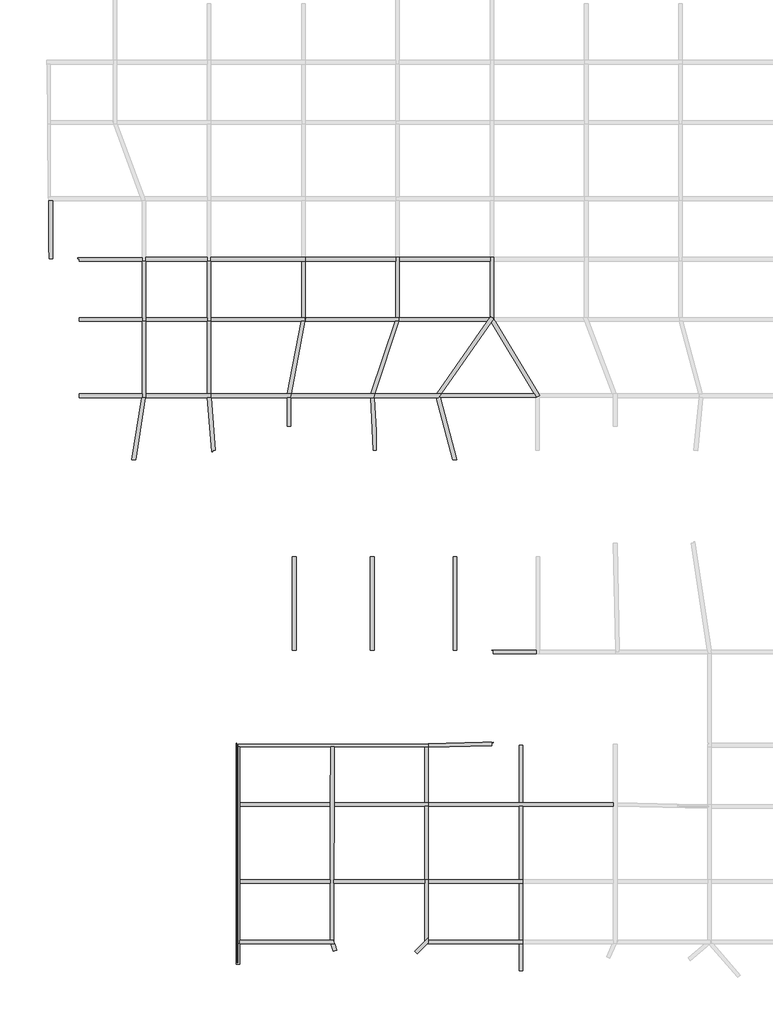
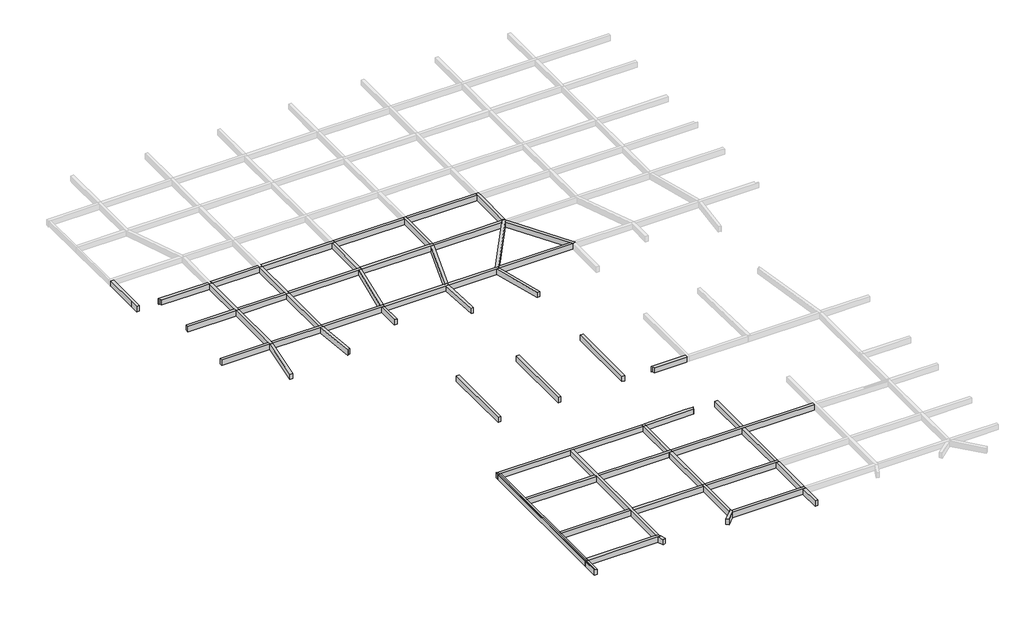
# One storey, part 1 of 15: 57 beams.
"""IFC4 building model written with IfcOpenShell, lengths in millimetres."""

from ifc_helpers import new_model, si_unit, frame, origin, place, context, project, spatial, polyline, outline, extrude, faceted_brep, element, save

model = new_model("IFC4")

# Units and contexts
model_context = context("Model", 3, world=origin())
ifc_project = project(units=[si_unit("LENGTHUNIT", "METRE", prefix="MILLI")], contexts=[model_context])

# Site, building, storey
site = spatial("IfcSite", under=ifc_project)
building = spatial("IfcBuilding", under=site)
storey = spatial("IfcBuildingStorey", under=building, Name="层高", Elevation=3300.0)

# Beams
placement = place(None, origin())
element("IfcBeam", 1, ObjectType="混凝土 - 矩形梁 : KL_beam", at=placement, inside=storey, context=model_context, shape_type="Brep", body=[
    faceted_brep([(117908.7029725, 38177.5268795, 3300.0), (117908.7029725, 38177.5268795, 2700.0), (118120.8350069, 37965.3948451, 2700.0), (118120.8350069, 37965.3948451, 3300.0), (118962.3353106, 38806.8951488, 3300.0), (119050.2032763, 38894.7631145, 3300.0), (119050.2032763, 39106.8951488, 3300.0), (119050.2032763, 39319.0271832, 3300.0), (118750.2032763, 39019.0271832, 3300.0), (118962.3353106, 38806.8951488, 2700.0), (119050.2032763, 38894.7631145, 2700.0), (118750.2032763, 39019.0271832, 2700.0), (119050.2032763, 39319.0271832, 2700.0), (119050.2032763, 39106.8951488, 2700.0)], [[[0, 1, 2, 3]], [[0, 3, 4, 5, 6, 7, 8]], [[3, 2, 9, 10, 5, 4]], [[2, 1, 11, 12, 13, 10, 9]], [[1, 0, 8, 7, 12, 11]], [[7, 6, 5, 10, 13, 12]]]),
])
element("IfcBeam", 2, ObjectType="混凝土 - 矩形梁 : KL_beam", at=placement, inside=storey, context=model_context, shape_type="Brep", body=[
    faceted_brep([(119050.2032763, 44092.5925365, 3300.0), (118750.2032763, 44092.5925365, 3300.0), (118750.2032763, 43792.5925365, 3300.0), (118750.2032763, 39019.0271832, 3300.0), (119050.2032763, 39319.0271832, 3300.0), (119050.2032763, 43792.5925365, 3300.0), (119050.2032763, 44092.5925365, 2700.0), (119050.2032763, 39319.0271832, 2700.0), (119050.2032763, 43792.5925365, 2700.0), (118750.2032763, 44092.5925365, 2700.0), (118750.2032763, 39019.0271832, 2700.0), (118750.2032763, 43792.5925365, 2700.0)], [[[0, 1, 2, 3, 4, 5]], [[6, 0, 5, 4, 7, 8]], [[9, 6, 8, 7, 10, 11]], [[1, 9, 11, 10, 3, 2]], [[4, 3, 10, 7]], [[1, 0, 6, 9]]]),
])
element("IfcBeam", 3, ObjectType="混凝土 - 矩形梁 : KL_beam", at=placement, inside=storey, context=model_context, shape_type="Brep", body=[
    faceted_brep([(118962.3353106, 38806.8951488, 3300.0), (118962.3353106, 38806.8951488, 2700.0), (126550.2032763, 38806.8951488, 2700.0), (126850.2032763, 38806.8951488, 2700.0), (126850.2032763, 38806.8951488, 3300.0), (126550.2032763, 38806.8951488, 3300.0), (119050.2032763, 38894.7631145, 3300.0), (119050.2032763, 38894.7631145, 2700.0), (119050.2032763, 39106.8951488, 3300.0), (119050.2032763, 39106.8951488, 2700.0), (126850.2032763, 39106.8951488, 3300.0), (126550.2032763, 39106.8951488, 3300.0), (126550.2032763, 39106.8951488, 2700.0), (126850.2032763, 39106.8951488, 2700.0)], [[[0, 1, 2, 3, 4, 5]], [[6, 7, 1, 0]], [[7, 6, 8, 9]], [[6, 0, 5, 4, 10, 11, 8]], [[1, 7, 9, 12, 13, 3, 2]], [[9, 8, 11, 10, 13, 12]], [[10, 4, 3, 13]]]),
])
element("IfcBeam", 4, ObjectType="混凝土 - 矩形梁 : KL_beam", at=placement, inside=storey, context=model_context, shape_type="Brep", body=[
    faceted_brep([(103150.2032763, 55392.5925366, 3300.0), (103150.2032763, 55092.5925366, 3300.0), (103172.8784474, 55092.5925366, 3300.0), (103172.8784474, 55392.5925366, 3300.0), (103150.2032763, 55392.5925366, 2700.0), (103172.8784474, 55392.5925366, 2700.0), (103150.2032763, 55092.5925366, 2700.0), (103172.8784474, 55092.5925366, 2700.0)], [[[0, 1, 2, 3]], [[4, 0, 3, 5]], [[6, 4, 5, 7]], [[1, 6, 7, 2]], [[1, 0, 4, 6]], [[3, 2, 7, 5]]]),
    faceted_brep([(119050.2032763, 55092.5925366, 3300.0), (119050.2032763, 55092.5925366, 2700.0), (119050.2032763, 55336.6611358, 2700.0), (119050.2032763, 55336.6611358, 3300.0), (103292.8784474, 55092.5925366, 2700.0), (103292.8784474, 55092.5925366, 3300.0), (103292.8784474, 55332.5925366, 3300.0), (103292.8784474, 55332.5925366, 2700.0), (103450.2032763, 55092.5925366, 3300.0), (110949.9406263, 55092.5925366, 3300.0), (111249.9410854, 55092.5925366, 3300.0), (118901.021306, 55332.5925366, 3300.0), (118901.021306, 55332.5925366, 2700.0), (111249.9410854, 55092.5925366, 2700.0), (110949.9406263, 55092.5925366, 2700.0), (103450.2032763, 55092.5925366, 2700.0)], [[[0, 1, 2, 3]], [[4, 5, 6, 7]], [[6, 5, 8, 9, 10, 0, 3, 11]], [[4, 7, 12, 2, 1, 13, 14, 15]], [[1, 0, 10, 9, 8, 5, 4, 15, 14, 13]], [[7, 6, 11, 12]], [[3, 2, 12, 11]]]),
])
element("IfcBeam", 5, ObjectType="混凝土 - 矩形梁 : KL_beam", at=placement, inside=storey, context=model_context, shape_type="Brep", body=[
    faceted_brep([(103450.2032763, 38806.8951488, 3300.0), (103450.2032763, 39106.8951488, 3300.0), (103450.2032763, 43792.5925365, 3300.0), (103450.2032763, 44092.5925365, 3300.0), (103450.2032763, 50192.5925366, 3300.0), (103450.2032763, 50492.5925366, 3300.0), (103450.2032763, 55092.5925366, 3300.0), (103292.8784474, 55092.5925366, 3300.0), (103292.8784474, 38806.8951488, 3300.0), (103450.2032763, 55092.5925366, 2700.0), (103450.2032763, 38806.8951488, 2700.0), (103450.2032763, 39106.8951488, 2700.0), (103450.2032763, 43792.5925365, 2700.0), (103450.2032763, 44092.5925365, 2700.0), (103450.2032763, 50192.5925366, 2700.0), (103450.2032763, 50492.5925366, 2700.0), (103292.8784474, 55092.5925366, 2700.0), (103292.8784474, 38806.8951488, 2700.0)], [[[0, 1, 2, 3, 4, 5, 6, 7, 8]], [[9, 6, 5, 4, 3, 2, 1, 0, 10, 11, 12, 13, 14, 15]], [[8, 7, 16, 17]], [[9, 15, 14, 13, 12, 11, 10, 17, 16]], [[6, 9, 16, 7]], [[10, 0, 8, 17]]]),
    faceted_brep([(103150.2032763, 55092.5925366, 3300.0), (103150.2032763, 55092.5925366, 2700.0), (103150.2032763, 38806.8951488, 2700.0), (103150.2032763, 38806.8951488, 3300.0), (103172.8784474, 55092.5925366, 2700.0), (103172.8784474, 38806.8951488, 2700.0), (103172.8784474, 55092.5925366, 3300.0), (103172.8784474, 38806.8951488, 3300.0)], [[[0, 1, 2, 3]], [[2, 1, 4, 5]], [[1, 0, 6, 4]], [[3, 2, 5, 7]], [[6, 7, 5, 4]], [[0, 3, 7, 6]]]),
])
element("IfcBeam", 6, ObjectType="混凝土 - 矩形梁 : KL_beam", at=placement, inside=storey, context=model_context, shape_type="SweptSolid", body=[
    extrude(outline(polyline([(103450.2032763, 37131.5943874), (103150.2032763, 37131.5943874), (103150.2032763, 38806.8951488), (103172.8784474, 38806.8951488), (103172.8784474, 37194.4264136), (103292.8784474, 37191.4907698), (103292.8784474, 38806.8951488), (103450.2032763, 38806.8951488), (103450.2032763, 37131.5943874)])), frame((0.0, 0.0, 2700.0), z_axis=(0.0, 0.0, 1.0), x_axis=(1.0, 0.0, 0.0)), (0.0, 0.0, 1.0), 600.0),
])
element("IfcBeam", 7, ObjectType="混凝土 - 矩形梁 : KL_beam", at=placement, inside=storey, context=model_context, shape_type="Brep", body=[
    faceted_brep([(111284.8038396, 38806.8951488, 3300.0), (111221.7575553, 38982.8323121, 3300.0), (111177.3002006, 39106.8951488, 3300.0), (110921.9741403, 39106.8951488, 3300.0), (103450.2032763, 39106.8951488, 3300.0), (103450.2032763, 38806.8951488, 3300.0), (110966.1236984, 38806.8951488, 3300.0), (111284.8038396, 38806.8951488, 2700.0), (103450.2032763, 38806.8951488, 2700.0), (110966.1236984, 38806.8951488, 2700.0), (111177.3002006, 39106.8951488, 2700.0), (111221.7575553, 38982.8323121, 2700.0), (103450.2032763, 39106.8951488, 2700.0), (110921.9741403, 39106.8951488, 2700.0)], [[[0, 1, 2, 3, 4, 5, 6]], [[7, 0, 6, 5, 8, 9]], [[10, 11, 7, 9, 8, 12, 13]], [[2, 10, 13, 12, 4, 3]], [[5, 4, 12, 8]], [[2, 1, 0, 7, 11, 10]]]),
])
element("IfcBeam", 8, ObjectType="混凝土 - 矩形梁 : KL_beam", at=placement, inside=storey, context=model_context, shape_type="SweptSolid", body=[
    extrude(outline(polyline([(111471.66124, 38285.4502876), (111189.2464034, 38184.2482122), (110966.1236984, 38806.8951488), (111284.8038396, 38806.8951488), (111471.66124, 38285.4502876)])), frame((0.0, 0.0, 2700.0), z_axis=(0.0, 0.0, 1.0), x_axis=(1.0, 0.0, 0.0)), (0.0, 0.0, 1.0), 600.0),
])
element("IfcBeam", 9, ObjectType="混凝土 - 矩形梁 : KL_beam", at=placement, inside=storey, context=model_context, shape_type="Brep", body=[
    faceted_brep([(110921.9741403, 39106.8951488, 3300.0), (111177.3002006, 39106.8951488, 3300.0), (111221.7575553, 38982.8323121, 3300.0), (111230.1720829, 43792.5925365, 3300.0), (111230.6969237, 44092.5925365, 3300.0), (111241.3686861, 50192.5925366, 3300.0), (111241.8935269, 50492.5925366, 3300.0), (111249.9410854, 55092.5925366, 3300.0), (110949.9406263, 55092.5925366, 3300.0), (110941.8930678, 50492.5925366, 3300.0), (110941.368227, 50192.5925366, 3300.0), (110930.6964646, 44092.5925365, 3300.0), (110930.1716238, 43792.5925365, 3300.0), (111221.7575553, 38982.8323121, 2700.0), (111230.1720829, 43792.5925365, 2700.0), (111230.6969237, 44092.5925365, 2700.0), (111241.3686861, 50192.5925366, 2700.0), (111241.8935269, 50492.5925366, 2700.0), (111249.9410854, 55092.5925366, 2700.0), (111177.3002006, 39106.8951488, 2700.0), (110921.9741403, 39106.8951488, 2700.0), (110930.1716238, 43792.5925365, 2700.0), (110930.6964646, 44092.5925365, 2700.0), (110941.368227, 50192.5925366, 2700.0), (110941.8930678, 50492.5925366, 2700.0), (110949.9406263, 55092.5925366, 2700.0)], [[[0, 1, 2, 3, 4, 5, 6, 7, 8, 9, 10, 11, 12]], [[2, 13, 14, 15, 16, 17, 18, 7, 6, 5, 4, 3]], [[19, 20, 21, 22, 23, 24, 25, 18, 17, 16, 15, 14, 13]], [[20, 0, 12, 11, 10, 9, 8, 25, 24, 23, 22, 21]], [[19, 1, 0, 20]], [[1, 19, 13, 2]], [[8, 7, 18, 25]]]),
])
element("IfcBeam", 10, ObjectType="混凝土 - 矩形梁 : KL_beam", at=placement, inside=storey, context=model_context, shape_type="Brep", body=[
    faceted_brep([(119050.2032763, 50192.5925366, 3300.0), (119050.2032763, 50467.5925366, 3300.0), (119050.2032763, 50492.5925366, 3300.0), (118750.2032763, 50492.5925366, 3300.0), (111241.8935269, 50492.5925366, 3300.0), (111241.3686861, 50192.5925366, 3300.0), (118750.2032763, 50192.5925366, 3300.0), (119050.2032763, 50192.5925366, 2700.0), (111241.3686861, 50192.5925366, 2700.0), (118750.2032763, 50192.5925366, 2700.0), (119050.2032763, 50492.5925366, 2700.0), (119050.2032763, 50467.5925366, 2700.0), (111241.8935269, 50492.5925366, 2700.0), (118750.2032763, 50492.5925366, 2700.0)], [[[0, 1, 2, 3, 4, 5, 6]], [[7, 0, 6, 5, 8, 9]], [[10, 11, 7, 9, 8, 12, 13]], [[2, 10, 13, 12, 4, 3]], [[5, 4, 12, 8]], [[2, 1, 0, 7, 11, 10]]]),
    faceted_brep([(103450.2032763, 50192.5925366, 3300.0), (103450.2032763, 50492.5925366, 3300.0), (103450.2032763, 50492.5925366, 2700.0), (103450.2032763, 50192.5925366, 2700.0), (110941.8930678, 50492.5925366, 3300.0), (110941.368227, 50192.5925366, 3300.0), (110941.368227, 50192.5925366, 2700.0), (110941.8930678, 50492.5925366, 2700.0)], [[[0, 1, 2, 3]], [[4, 5, 6, 7]], [[1, 0, 5, 4]], [[0, 3, 6, 5]], [[3, 2, 7, 6]], [[2, 1, 4, 7]]]),
])
element("IfcBeam", 11, ObjectType="混凝土 - 矩形梁 : KL_beam", at=placement, inside=storey, context=model_context, shape_type="SweptSolid", body=[
    extrude(outline(polyline([(103450.2032763, 43792.5925365), (103450.2032763, 44092.5925365), (110930.6964646, 44092.5925365), (110930.1716238, 43792.5925365), (103450.2032763, 43792.5925365)])), frame((0.0, 0.0, 2700.0), z_axis=(0.0, 0.0, 1.0), x_axis=(1.0, 0.0, 0.0)), (0.0, 0.0, 1.0), 600.0),
    extrude(outline(polyline([(118750.2032763, 44092.5925365), (118750.2032763, 43792.5925365), (111230.1720829, 43792.5925365), (111230.6969237, 44092.5925365), (118750.2032763, 44092.5925365)])), frame((0.0, 0.0, 2700.0), z_axis=(0.0, 0.0, 1.0), x_axis=(1.0, 0.0, 0.0)), (0.0, 0.0, 1.0), 600.0),
])
element("IfcBeam", 12, ObjectType="混凝土 - 矩形梁 : KL_beam", at=placement, inside=storey, context=model_context, shape_type="Brep", body=[
    faceted_brep([(134350.2032763, 50167.5925366, 3300.0), (134350.2032763, 50467.5925366, 3300.0), (126850.2032763, 50467.5925366, 3300.0), (126550.2032763, 50467.5925366, 3300.0), (119050.2032763, 50467.5925366, 3300.0), (119050.2032763, 50192.5925366, 3300.0), (118750.2032763, 50192.5925366, 3300.0), (118750.2032763, 50167.5925366, 3300.0), (119050.2032763, 50167.5925366, 3300.0), (126550.2032763, 50167.5925366, 3300.0), (126850.2032763, 50167.5925366, 3300.0), (134350.2032763, 50167.5925366, 2700.0), (118750.2032763, 50167.5925366, 2700.0), (119050.2032763, 50167.5925366, 2700.0), (126550.2032763, 50167.5925366, 2700.0), (126850.2032763, 50167.5925366, 2700.0), (134350.2032763, 50467.5925366, 2700.0), (118750.2032763, 50192.5925366, 2700.0), (119050.2032763, 50192.5925366, 2700.0), (119050.2032763, 50467.5925366, 2700.0), (126550.2032763, 50467.5925366, 2700.0), (126850.2032763, 50467.5925366, 2700.0)], [[[0, 1, 2, 3, 4, 5, 6, 7, 8, 9, 10]], [[11, 0, 10, 9, 8, 7, 12, 13, 14, 15]], [[16, 11, 15, 14, 13, 12, 17, 18, 19, 20, 21]], [[1, 16, 21, 20, 19, 4, 3, 2]], [[1, 0, 11, 16]], [[5, 18, 17, 6]], [[12, 7, 6, 17]], [[18, 5, 4, 19]]]),
])
element("IfcBeam", 13, ObjectType="混凝土 - 矩形梁 : KL_beam", at=placement, inside=storey, context=model_context, shape_type="Brep", body=[
    faceted_brep([(126850.2032763, 43792.5925365, 3300.0), (126850.2032763, 44092.5925365, 3300.0), (126550.2032763, 44092.5925365, 3300.0), (119050.2032763, 44092.5925365, 3300.0), (119050.2032763, 43792.5925365, 3300.0), (126550.2032763, 43792.5925365, 3300.0), (126850.2032763, 43792.5925365, 2700.0), (119050.2032763, 43792.5925365, 2700.0), (126550.2032763, 43792.5925365, 2700.0), (126850.2032763, 44092.5925365, 2700.0), (119050.2032763, 44092.5925365, 2700.0), (126550.2032763, 44092.5925365, 2700.0)], [[[0, 1, 2, 3, 4, 5]], [[6, 0, 5, 4, 7, 8]], [[9, 6, 8, 7, 10, 11]], [[1, 9, 11, 10, 3, 2]], [[4, 3, 10, 7]], [[1, 0, 6, 9]]]),
])
element("IfcBeam", 14, ObjectType="混凝土 - 矩形梁 : KL_beam", at=placement, inside=storey, context=model_context, shape_type="SweptSolid", body=[
    extrude(outline(polyline([(126850.2032763, 36559.4144068), (126550.2032763, 36559.4144068), (126550.2032763, 38806.8951488), (126850.2032763, 38806.8951488), (126850.2032763, 36559.4144068)])), frame((0.0, 0.0, 2700.0), z_axis=(0.0, 0.0, 1.0), x_axis=(1.0, 0.0, 0.0)), (0.0, 0.0, 1.0), 600.0),
])
element("IfcBeam", 15, ObjectType="混凝土 - 矩形梁 : KL_beam", at=placement, inside=storey, context=model_context, shape_type="SweptSolid", body=[
    extrude(outline(polyline([(126850.2032763, 39106.8951488), (126550.2032763, 39106.8951488), (126550.2032763, 43792.5925365), (126850.2032763, 43792.5925365), (126850.2032763, 39106.8951488)])), frame((0.0, 0.0, 2700.0), z_axis=(0.0, 0.0, 1.0), x_axis=(1.0, 0.0, 0.0)), (0.0, 0.0, 1.0), 600.0),
])
element("IfcBeam", 16, ObjectType="混凝土 - 矩形梁 : KL_beam", at=placement, inside=storey, context=model_context, shape_type="SweptSolid", body=[
    extrude(outline(polyline([(126850.2032763, 44092.5925365), (126550.2032763, 44092.5925365), (126550.2032763, 50167.5925366), (126850.2032763, 50167.5925366), (126850.2032763, 44092.5925365)])), frame((0.0, 0.0, 2700.0), z_axis=(0.0, 0.0, 1.0), x_axis=(1.0, 0.0, 0.0)), (0.0, 0.0, 1.0), 600.0),
])
element("IfcBeam", 17, ObjectType="混凝土 - 矩形梁 : KL_beam", at=placement, inside=storey, context=model_context, shape_type="SweptSolid", body=[
    extrude(outline(polyline([(119050.2032763, 44092.5925365), (118750.2032763, 44092.5925365), (118750.2032763, 50167.5925366), (119050.2032763, 50167.5925366), (119050.2032763, 44092.5925365)])), frame((0.0, 0.0, 2700.0), z_axis=(0.0, 0.0, 1.0), x_axis=(1.0, 0.0, 0.0)), (0.0, 0.0, 1.0), 600.0),
])
element("IfcBeam", 18, ObjectType="混凝土 - 矩形梁 : KL_beam", at=placement, inside=storey, context=model_context, shape_type="Brep", body=[
    faceted_brep([(118750.2032763, 50492.5925366, 3300.0), (119050.2032763, 50492.5925366, 3300.0), (119050.2032763, 55085.0391316, 3300.0), (119050.2032763, 55336.6611358, 3300.0), (118901.021306, 55332.5925366, 3300.0), (118750.2032763, 55332.5925366, 3300.0), (119050.2032763, 50492.5925366, 2700.0), (119050.2032763, 55085.0391316, 2700.0), (119050.2032763, 55336.6611358, 2700.0), (118750.2032763, 50492.5925366, 2700.0), (118750.2032763, 55332.5925366, 2700.0), (118901.021306, 55332.5925366, 2700.0)], [[[0, 1, 2, 3, 4, 5]], [[1, 6, 7, 8, 3, 2]], [[6, 9, 10, 11, 8, 7]], [[9, 0, 5, 10]], [[1, 0, 9, 6]], [[5, 4, 11, 10]], [[4, 3, 8, 11]]]),
])
element("IfcBeam", 19, ObjectType="混凝土 - 矩形梁 : KL_beam", at=placement, inside=storey, context=model_context, shape_type="Brep", body=[
    faceted_brep([(124375.3504625, 55452.5925367, 3300.0), (124389.4925981, 55452.5925367, 3300.0), (124389.4925981, 55466.7346723, 3300.0), (124389.4925981, 55452.5925367, 2700.0), (124375.3504625, 55452.5925367, 2700.0), (124389.4925981, 55466.7346723, 2700.0)], [[[0, 1, 2]], [[3, 4, 5]], [[1, 3, 5, 2]], [[1, 0, 4, 3]], [[0, 2, 5, 4]]]),
    faceted_brep([(124263.235473, 55170.7719197, 3300.0), (119050.2032763, 55085.0391316, 3300.0), (119050.2032763, 55085.0391316, 2700.0), (124263.235473, 55170.7719197, 2700.0), (124269.4925981, 55470.9153906, 3300.0), (124269.4925981, 55470.9153906, 2700.0), (123522.2775593, 55458.6267981, 2700.0), (123522.2775593, 55458.6267981, 3300.0), (124269.4925981, 55177.0290448, 3300.0), (124269.4925981, 55177.0290448, 2700.0), (119050.2032763, 55092.5925366, 3300.0), (119050.2032763, 55336.6611358, 3300.0), (119050.2032763, 55336.6611358, 2700.0), (119050.2032763, 55092.5925366, 2700.0)], [[[0, 1, 2, 3]], [[4, 5, 6, 7]], [[5, 4, 8, 9]], [[2, 1, 10, 11, 12, 13]], [[1, 0, 8, 4, 7, 11, 10]], [[3, 2, 13, 12, 6, 5, 9]], [[7, 6, 12, 11]], [[0, 3, 9, 8]]]),
])
element("IfcBeam", 20, ObjectType="混凝土 - 矩形梁 : KL_beam", at=placement, inside=storey, context=model_context, shape_type="SweptSolid", body=[
    extrude(outline(polyline([(100750.3009381, 95592.1233035), (100750.3009381, 95292.1233035), (95650.3009362, 95292.1233035), (95650.3009362, 95592.1233035), (100750.3009381, 95592.1233035)])), frame((0.0, 0.0, 2700.0), z_axis=(0.0, 0.0, 1.0), x_axis=(1.0, 0.0, 0.0)), (0.0, 0.0, 1.0), 600.0),
])
element("IfcBeam", 21, ObjectType="混凝土 - 矩形梁 : KL_beam", at=placement, inside=storey, context=model_context, shape_type="Brep", body=[
    faceted_brep([(108850.3009381, 95292.1233035, 3300.0), (108850.3009381, 95592.1233035, 3300.0), (108550.3009381, 95592.1233035, 3300.0), (101050.3009381, 95592.1233035, 3300.0), (101050.3009381, 95292.1233035, 3300.0), (108550.3009381, 95292.1233035, 3300.0), (108850.3009381, 95292.1233035, 2700.0), (101050.3009381, 95292.1233035, 2700.0), (108550.3009381, 95292.1233035, 2700.0), (108850.3009381, 95592.1233035, 2700.0), (101050.3009381, 95592.1233035, 2700.0), (108550.3009381, 95592.1233035, 2700.0)], [[[0, 1, 2, 3, 4, 5]], [[6, 0, 5, 4, 7, 8]], [[9, 6, 8, 7, 10, 11]], [[1, 9, 11, 10, 3, 2]], [[4, 3, 10, 7]], [[1, 0, 6, 9]]]),
])
element("IfcBeam", 22, ObjectType="混凝土 - 矩形梁 : KL_beam", at=placement, inside=storey, context=model_context, shape_type="Brep", body=[
    faceted_brep([(100750.3009381, 90292.3894162, 3300.0), (101050.3009381, 90292.3894162, 3300.0), (101050.3009381, 90592.3894162, 3300.0), (101050.3009381, 95292.1233035, 3300.0), (100750.3009381, 95292.1233035, 3300.0), (100750.3009381, 90592.3894162, 3300.0), (101050.3009381, 90292.3894162, 2700.0), (101050.3009381, 90592.3894162, 2700.0), (101050.3009381, 95292.1233035, 2700.0), (100750.3009381, 90292.3894162, 2700.0), (100750.3009381, 90592.3894162, 2700.0), (100750.3009381, 95292.1233035, 2700.0)], [[[0, 1, 2, 3, 4, 5]], [[1, 6, 7, 8, 3, 2]], [[6, 9, 10, 11, 8, 7]], [[9, 0, 5, 4, 11, 10]], [[4, 3, 8, 11]], [[1, 0, 9, 6]]]),
])
element("IfcBeam", 23, ObjectType="混凝土 - 矩形梁 : KL_beam", at=placement, inside=storey, context=model_context, shape_type="Brep", body=[
    faceted_brep([(95350.3009362, 90292.3894162, 3300.0), (95650.3009362, 90292.3894162, 3300.0), (95650.3009362, 90592.3894162, 3300.0), (95650.3009362, 95292.1233035, 3300.0), (95350.3009362, 95292.1233035, 3300.0), (95350.3009362, 95267.3846604, 3300.0), (95350.3009362, 90592.3894162, 3300.0), (95650.3009362, 90292.3894162, 2700.0), (95650.3009362, 90592.3894162, 2700.0), (95650.3009362, 95292.1233035, 2700.0), (95350.3009362, 90292.3894162, 2700.0), (95350.3009362, 90592.3894162, 2700.0), (95350.3009362, 95267.3846604, 2700.0), (95350.3009362, 95292.1233035, 2700.0)], [[[0, 1, 2, 3, 4, 5, 6]], [[1, 7, 8, 9, 3, 2]], [[7, 10, 11, 12, 13, 9, 8]], [[10, 0, 6, 5, 4, 13, 12, 11]], [[4, 3, 9, 13]], [[1, 0, 10, 7]]]),
])
element("IfcBeam", 24, ObjectType="混凝土 - 矩形梁 : KL_beam", at=placement, inside=storey, context=model_context, shape_type="SweptSolid", body=[
    extrude(outline(polyline([(100750.3009381, 90592.3894162), (100750.3009381, 90292.3894162), (95650.3009362, 90292.3894162), (95650.3009362, 90592.3894162), (100750.3009381, 90592.3894162)])), frame((0.0, 0.0, 2700.0), z_axis=(0.0, 0.0, 1.0), x_axis=(1.0, 0.0, 0.0)), (0.0, 0.0, 1.0), 600.0),
])
element("IfcBeam", 25, ObjectType="混凝土 - 矩形梁 : KL_beam", at=placement, inside=storey, context=model_context, shape_type="Brep", body=[
    faceted_brep([(108850.3009381, 90292.3894162, 3300.0), (108850.3009381, 90428.2293199, 3300.0), (108850.3009381, 90592.3894162, 3300.0), (108550.3009381, 90592.3894162, 3300.0), (101050.3009381, 90592.3894162, 3300.0), (101050.3009381, 90292.3894162, 3300.0), (108519.0286184, 90292.3894162, 3300.0), (108824.4235843, 90292.3894162, 3300.0), (108850.3009381, 90292.3894162, 2700.0), (101050.3009381, 90292.3894162, 2700.0), (108519.0286184, 90292.3894162, 2700.0), (108824.4235843, 90292.3894162, 2700.0), (108850.3009381, 90592.3894162, 2700.0), (108850.3009381, 90428.2293199, 2700.0), (101050.3009381, 90592.3894162, 2700.0), (108550.3009381, 90592.3894162, 2700.0)], [[[0, 1, 2, 3, 4, 5, 6, 7]], [[8, 0, 7, 6, 5, 9, 10, 11]], [[12, 13, 8, 11, 10, 9, 14, 15]], [[2, 12, 15, 14, 4, 3]], [[5, 4, 14, 9]], [[2, 1, 0, 8, 13, 12]]]),
])
element("IfcBeam", 26, ObjectType="混凝土 - 矩形梁 : KL_beam", at=placement, inside=storey, context=model_context, shape_type="SweptSolid", body=[
    extrude(outline(polyline([(108550.3009381, 95292.1233035), (108850.3009381, 95292.1233035), (108850.3009381, 90592.3894162), (108550.3009381, 90592.3894162), (108550.3009381, 95292.1233035)])), frame((0.0, 0.0, 2700.0), z_axis=(0.0, 0.0, 1.0), x_axis=(1.0, 0.0, 0.0)), (0.0, 0.0, 1.0), 600.0),
])
element("IfcBeam", 27, ObjectType="混凝土 - 矩形梁 : KL_beam", at=placement, inside=storey, context=model_context, shape_type="Brep", body=[
    faceted_brep([(95350.3009362, 83992.3894162, 3300.0), (95628.413039, 83992.3894162, 3300.0), (95650.3009362, 83992.3894162, 3300.0), (95650.3009362, 84292.3894162, 3300.0), (95650.3009362, 90292.3894162, 3300.0), (95350.3009362, 90292.3894162, 3300.0), (95350.3009362, 84292.3894162, 3300.0), (95350.3009362, 83992.3894162, 2700.0), (95350.3009362, 90292.3894162, 2700.0), (95350.3009362, 84292.3894162, 2700.0), (95650.3009362, 83992.3894162, 2700.0), (95628.413039, 83992.3894162, 2700.0), (95650.3009362, 90292.3894162, 2700.0), (95650.3009362, 84292.3894162, 2700.0)], [[[0, 1, 2, 3, 4, 5, 6]], [[7, 0, 6, 5, 8, 9]], [[10, 11, 7, 9, 8, 12, 13]], [[2, 10, 13, 12, 4, 3]], [[5, 4, 12, 8]], [[2, 1, 0, 7, 11, 10]]]),
])
element("IfcBeam", 28, ObjectType="混凝土 - 矩形梁 : KL_beam", at=placement, inside=storey, context=model_context, shape_type="Brep", body=[
    faceted_brep([(101050.3009381, 83992.3894162, 3300.0), (101050.3009381, 84292.3894162, 3300.0), (100750.3009381, 84292.3894162, 3300.0), (95650.3009362, 84292.3894162, 3300.0), (95650.3009362, 83992.3894162, 3300.0), (100761.9515162, 83992.3894162, 3300.0), (101050.3009381, 83992.3894162, 2700.0), (95650.3009362, 83992.3894162, 2700.0), (100761.9515162, 83992.3894162, 2700.0), (101050.3009381, 84292.3894162, 2700.0), (95650.3009362, 84292.3894162, 2700.0), (100750.3009381, 84292.3894162, 2700.0)], [[[0, 1, 2, 3, 4, 5]], [[6, 0, 5, 4, 7, 8]], [[9, 6, 8, 7, 10, 11]], [[1, 9, 11, 10, 3, 2]], [[4, 3, 10, 7]], [[1, 0, 6, 9]]]),
])
element("IfcBeam", 29, ObjectType="混凝土 - 矩形梁 : KL_beam", at=placement, inside=storey, context=model_context, shape_type="SweptSolid", body=[
    extrude(outline(polyline([(100750.3009381, 90292.3894162), (101050.3009381, 90292.3894162), (101050.3009381, 84292.3894162), (100750.3009381, 84292.3894162), (100750.3009381, 90292.3894162)])), frame((0.0, 0.0, 2700.0), z_axis=(0.0, 0.0, 1.0), x_axis=(1.0, 0.0, 0.0)), (0.0, 0.0, 1.0), 600.0),
])
element("IfcBeam", 30, ObjectType="混凝土 - 矩形梁 : KL_beam", at=placement, inside=storey, context=model_context, shape_type="Brep", body=[
    faceted_brep([(107624.2804397, 83992.3894162, 3300.0), (107681.4301132, 84292.3894162, 3300.0), (107376.0351473, 84292.3894162, 3300.0), (101050.3009381, 84292.3894162, 3300.0), (101050.3009381, 83992.3894162, 3300.0), (101062.932626, 83992.3894162, 3300.0), (107350.1577935, 83992.3894162, 3300.0), (107624.2804397, 83992.3894162, 2700.0), (101050.3009381, 83992.3894162, 2700.0), (101062.932626, 83992.3894162, 2700.0), (107350.1577935, 83992.3894162, 2700.0), (107681.4301132, 84292.3894162, 2700.0), (101050.3009381, 84292.3894162, 2700.0), (107376.0351473, 84292.3894162, 2700.0)], [[[0, 1, 2, 3, 4, 5, 6]], [[7, 0, 6, 5, 4, 8, 9, 10]], [[11, 7, 10, 9, 8, 12, 13]], [[1, 11, 13, 12, 3, 2]], [[4, 3, 12, 8]], [[1, 0, 7, 11]]]),
])
element("IfcBeam", 31, ObjectType="混凝土 - 矩形梁 : KL_beam", at=placement, inside=storey, context=model_context, shape_type="Brep", body=[
    faceted_brep([(108850.3009381, 90592.3894162, 3300.0), (108850.3009381, 90428.2293199, 3300.0), (108881.5732578, 90592.3894162, 3300.0), (108850.3009381, 90428.2293199, 2700.0), (108881.5732578, 90592.3894162, 2700.0), (108850.3009381, 90592.3894162, 2700.0)], [[[0, 1, 2]], [[1, 3, 4, 2]], [[3, 5, 4]], [[5, 0, 2, 4]], [[1, 0, 5, 3]]]),
    faceted_brep([(108519.0286184, 90292.3894162, 3300.0), (108519.0286184, 90292.3894162, 2700.0), (107376.0351473, 84292.3894162, 2700.0), (107376.0351473, 84292.3894162, 3300.0), (108824.4235843, 90292.3894162, 3300.0), (108824.4235843, 90292.3894162, 2700.0), (108550.3009381, 90292.3894162, 2700.0), (108550.3009381, 90292.3894162, 3300.0), (107681.4301132, 84292.3894162, 2700.0), (107681.4301132, 84292.3894162, 3300.0)], [[[0, 1, 2, 3]], [[4, 5, 6, 1, 0, 7]], [[3, 2, 8, 9]], [[7, 0, 3, 9, 4]], [[5, 4, 9, 8]], [[6, 5, 8, 2, 1]]]),
])
element("IfcBeam", 32, ObjectType="混凝土 - 矩形梁 : KL_beam", at=placement, inside=storey, context=model_context, shape_type="Brep", body=[
    faceted_brep([(107681.4301132, 84292.3894162, 3300.0), (107624.2804397, 83992.3894162, 3300.0), (107650.1577935, 83992.3894162, 3300.0), (114256.2034762, 83992.3894162, 3300.0), (114506.2541434, 83992.3894162, 3300.0), (114606.3553849, 84292.3894162, 3300.0), (114290.0955889, 84292.3894162, 3300.0), (107624.2804397, 83992.3894162, 2700.0), (107650.1577935, 83992.3894162, 2700.0), (114256.2034762, 83992.3894162, 2700.0), (114506.2541434, 83992.3894162, 2700.0), (107681.4301132, 84292.3894162, 2700.0), (114290.0955889, 84292.3894162, 2700.0), (114606.3553849, 84292.3894162, 2700.0)], [[[0, 1, 2, 3, 4, 5, 6]], [[1, 7, 8, 9, 10, 4, 3, 2]], [[7, 11, 12, 13, 10, 9, 8]], [[11, 0, 6, 5, 13, 12]], [[1, 0, 11, 7]], [[5, 4, 10, 13]]]),
])
element("IfcBeam", 33, ObjectType="混凝土 - 矩形梁 : KL_beam", at=placement, inside=storey, context=model_context, shape_type="Brep", body=[
    faceted_brep([(107350.1577935, 81640.79875, 3300.0), (107650.1577935, 81640.79875, 3300.0), (107650.1577935, 83992.3894162, 3300.0), (107624.2804397, 83992.3894162, 3300.0), (107350.1577935, 83992.3894162, 3300.0), (107350.1577935, 81640.79875, 2700.0), (107350.1577935, 83992.3894162, 2700.0), (107650.1577935, 81640.79875, 2700.0), (107624.2804397, 83992.3894162, 2700.0), (107650.1577935, 83992.3894162, 2700.0)], [[[0, 1, 2, 3, 4]], [[5, 0, 4, 6]], [[7, 5, 6, 8, 9]], [[1, 7, 9, 2]], [[1, 0, 5, 7]], [[2, 9, 8, 6, 4, 3]]]),
])
element("IfcBeam", 34, ObjectType="混凝土 - 矩形梁 : KL_beam", at=placement, inside=storey, context=model_context, shape_type="Brep", body=[
    faceted_brep([(108850.3009381, 90292.3894162, 3300.0), (116292.1204194, 90292.3894162, 3300.0), (116608.3802153, 90292.3894162, 3300.0), (116608.3802153, 90592.3894162, 3300.0), (116350.3009381, 90592.3894162, 3300.0), (108881.5732578, 90592.3894162, 3300.0), (108850.3009381, 90428.2293199, 3300.0), (108850.3009381, 90292.3894162, 2700.0), (116292.1204194, 90292.3894162, 2700.0), (116608.3802153, 90292.3894162, 2700.0), (108850.3009381, 90428.2293199, 2700.0), (108881.5732578, 90592.3894162, 2700.0), (116350.3009381, 90592.3894162, 2700.0), (116608.3802153, 90592.3894162, 2700.0)], [[[0, 1, 2, 3, 4, 5, 6]], [[2, 1, 0, 7, 8, 9]], [[9, 8, 7, 10, 11, 12, 13]], [[3, 13, 12, 11, 5, 4]], [[7, 0, 6, 10]], [[6, 5, 11, 10]], [[3, 2, 9, 13]]]),
])
element("IfcBeam", 35, ObjectType="混凝土 - 矩形梁 : KL_beam", at=placement, inside=storey, context=model_context, shape_type="SweptSolid", body=[
    extrude(outline(polyline([(116608.3802153, 90292.3894162), (114606.3553849, 84292.3894162), (114290.0955889, 84292.3894162), (116292.1204194, 90292.3894162), (116608.3802153, 90292.3894162)])), frame((0.0, 0.0, 2700.0), z_axis=(0.0, 0.0, 1.0), x_axis=(1.0, 0.0, 0.0)), (0.0, 0.0, 1.0), 600.0),
])
element("IfcBeam", 36, ObjectType="混凝土 - 矩形梁 : KL_beam", at=placement, inside=storey, context=model_context, shape_type="Brep", body=[
    faceted_brep([(114606.3553849, 84292.3894162, 3300.0), (114506.2541434, 83992.3894162, 3300.0), (114556.6575013, 83992.3894162, 3300.0), (119709.1352634, 83992.3894162, 3300.0), (119878.3508221, 83992.3894162, 3300.0), (119895.8942689, 84017.4440548, 3300.0), (120088.4130836, 84292.3894162, 3300.0), (119722.1807069, 84292.3894162, 3300.0), (114506.2541434, 83992.3894162, 2700.0), (114556.6575013, 83992.3894162, 2700.0), (119709.1352634, 83992.3894162, 2700.0), (119878.3508221, 83992.3894162, 2700.0), (114606.3553849, 84292.3894162, 2700.0), (119722.1807069, 84292.3894162, 2700.0), (120088.4130836, 84292.3894162, 2700.0), (119895.8942689, 84017.4440548, 2700.0)], [[[0, 1, 2, 3, 4, 5, 6, 7]], [[1, 8, 9, 10, 11, 4, 3, 2]], [[8, 12, 13, 14, 15, 11, 10, 9]], [[12, 0, 7, 6, 14, 13]], [[1, 0, 12, 8]], [[6, 5, 4, 11, 15, 14]]]),
])
element("IfcBeam", 37, ObjectType="混凝土 - 矩形梁 : KL_beam", at=placement, inside=storey, context=model_context, shape_type="Brep", body=[
    faceted_brep([(124437.9977923, 90504.2401482, 3300.0), (124312.1075909, 90592.3894162, 3300.0), (124192.252179, 90676.3130791, 3300.0), (124150.1664518, 90616.2084317, 3300.0), (124133.4881976, 90592.3894162, 3300.0), (123923.4259362, 90292.3894162, 3300.0), (119722.1807069, 84292.3894162, 3300.0), (120088.4130836, 84292.3894162, 3300.0), (120105.9565304, 84317.4440548, 3300.0), (124249.6405196, 90235.2380846, 3300.0), (124437.9977923, 90504.2401482, 2700.0), (120088.4130836, 84292.3894162, 2700.0), (120105.9565304, 84317.4440548, 2700.0), (124249.6405196, 90235.2380846, 2700.0), (124192.252179, 90676.3130791, 2700.0), (124312.1075909, 90592.3894162, 2700.0), (119722.1807069, 84292.3894162, 2700.0), (123923.4259362, 90292.3894162, 2700.0), (124133.4881976, 90592.3894162, 2700.0), (124150.1664518, 90616.2084317, 2700.0)], [[[0, 1, 2, 3, 4, 5, 6, 7, 8, 9]], [[10, 0, 9, 8, 7, 11, 12, 13]], [[14, 15, 10, 13, 12, 11, 16, 17, 18, 19]], [[2, 14, 19, 18, 17, 16, 6, 5, 4, 3]], [[7, 6, 16, 11]], [[2, 1, 0, 10, 15, 14]]]),
])
element("IfcBeam", 38, ObjectType="混凝土 - 矩形梁 : KL_beam", at=placement, inside=storey, context=model_context, shape_type="Brep", body=[
    faceted_brep([(128242.8182795, 84171.9554773, 3300.0), (128220.534006, 84209.0427364, 3300.0), (128155.3999228, 84317.4440548, 3300.0), (124565.2905543, 90292.3894162, 3300.0), (124450.1664518, 90483.9880978, 3300.0), (124437.9977923, 90504.2401482, 3300.0), (124249.6405196, 90235.2380846, 3300.0), (127805.4099036, 84317.4440548, 3300.0), (127985.6680893, 84017.4440548, 3300.0), (128220.534006, 84158.5657349, 3300.0), (127985.6680893, 84017.4440548, 2700.0), (124249.6405196, 90235.2380846, 2700.0), (127805.4099036, 84317.4440548, 2700.0), (124437.9977923, 90504.2401482, 2700.0), (124450.1664518, 90483.9880978, 2700.0), (124565.2905543, 90292.3894162, 2700.0), (128155.3999228, 84317.4440548, 2700.0), (128220.534006, 84209.0427364, 2700.0), (128242.8182795, 84171.9554773, 2700.0), (128220.534006, 84158.5657349, 2700.0)], [[[0, 1, 2, 3, 4, 5, 6, 7, 8, 9]], [[10, 8, 7, 6, 11, 12]], [[13, 14, 15, 16, 17, 18, 19, 10, 12, 11]], [[5, 4, 3, 2, 1, 0, 18, 17, 16, 15, 14, 13]], [[6, 5, 13, 11]], [[0, 9, 8, 10, 19, 18]]]),
])
element("IfcBeam", 39, ObjectType="混凝土 - 矩形梁 : KL_beam", at=placement, inside=storey, context=model_context, shape_type="Brep", body=[
    faceted_brep([(119895.8942689, 84017.4440548, 3300.0), (120012.8941843, 84017.4440548, 3300.0), (127920.534006, 84017.4440548, 3300.0), (127985.6680893, 84017.4440548, 3300.0), (127805.4099036, 84317.4440548, 3300.0), (120105.9565304, 84317.4440548, 3300.0), (120088.4130836, 84292.3894162, 3300.0), (120105.9565304, 84317.4440548, 2700.0), (127805.4099036, 84317.4440548, 2700.0), (127985.6680893, 84017.4440548, 2700.0), (127920.534006, 84017.4440548, 2700.0), (120012.8941843, 84017.4440548, 2700.0), (119895.8942689, 84017.4440548, 2700.0), (120088.4130836, 84292.3894162, 2700.0)], [[[0, 1, 2, 3, 4, 5, 6]], [[7, 5, 4, 8]], [[9, 10, 11, 12, 13, 7, 8]], [[3, 2, 1, 0, 12, 11, 10, 9]], [[12, 0, 6, 5, 7, 13]], [[4, 3, 9, 8]]]),
])
element("IfcBeam", 40, ObjectType="混凝土 - 矩形梁 : KL_beam", at=placement, inside=storey, context=model_context, shape_type="Brep", body=[
    faceted_brep([(124437.9977923, 90504.2401482, 3300.0), (124385.0323686, 90592.3894162, 3300.0), (124312.1075909, 90592.3894162, 3300.0), (124385.0323686, 90592.3894162, 2700.0), (124437.9977923, 90504.2401482, 2700.0), (124312.1075909, 90592.3894162, 2700.0)], [[[0, 1, 2]], [[3, 4, 5]], [[1, 3, 5, 2]], [[3, 1, 0, 4]], [[0, 2, 5, 4]]]),
    faceted_brep([(116608.3802153, 90292.3894162, 3300.0), (116608.3802153, 90292.3894162, 2700.0), (123923.4259362, 90292.3894162, 2700.0), (123923.4259362, 90292.3894162, 3300.0), (116608.3802153, 90592.3894162, 3300.0), (116608.3802153, 90592.3894162, 2700.0), (124133.4881976, 90592.3894162, 2700.0), (124133.4881976, 90592.3894162, 3300.0), (116650.3009381, 90592.3894162, 3300.0), (116650.3009381, 90592.3894162, 2700.0)], [[[0, 1, 2, 3]], [[0, 4, 5, 1]], [[3, 2, 6, 7]], [[4, 0, 3, 7, 8]], [[1, 5, 9, 6, 2]], [[5, 4, 8, 7, 6, 9]]]),
])
element("IfcBeam", 41, ObjectType="混凝土 - 矩形梁 : KL_beam", at=placement, inside=storey, context=model_context, shape_type="Brep", body=[
    faceted_brep([(116350.3009381, 90592.3894162, 3300.0), (116608.3802153, 90592.3894162, 3300.0), (116650.3009381, 90592.3894162, 3300.0), (116650.3009381, 95292.1233035, 3300.0), (116650.3009381, 95592.1233035, 3300.0), (116350.3009381, 95592.1233035, 3300.0), (116350.3009381, 95292.1233035, 3300.0), (116650.3009381, 95592.1233035, 2700.0), (116650.3009381, 90592.3894162, 2700.0), (116650.3009381, 95292.1233035, 2700.0), (116608.3802153, 90592.3894162, 2700.0), (116350.3009381, 90592.3894162, 2700.0), (116350.3009381, 95292.1233035, 2700.0), (116350.3009381, 95592.1233035, 2700.0)], [[[0, 1, 2, 3, 4, 5, 6]], [[7, 4, 3, 2, 8, 9]], [[8, 10, 11, 12, 13, 7, 9]], [[11, 0, 6, 5, 13, 12]], [[0, 11, 10, 8, 2, 1]], [[5, 4, 7, 13]]]),
])
element("IfcBeam", 42, ObjectType="混凝土 - 矩形梁 : KL_beam", at=placement, inside=storey, context=model_context, shape_type="Brep", body=[
    faceted_brep([(124450.1664518, 90483.9880978, 3300.0), (124450.1664518, 90483.9880978, 2700.0), (124450.1664518, 90592.3894162, 2700.0), (124450.1664518, 95292.1233035, 2700.0), (124450.1664518, 95592.1233035, 2700.0), (124450.1664518, 95592.1233035, 3300.0), (124450.1664518, 95292.1233035, 3300.0), (124450.1664518, 90592.3894162, 3300.0), (124385.0323686, 90592.3894162, 3300.0), (124385.0323686, 90592.3894162, 2700.0), (124437.9977923, 90504.2401482, 2700.0), (124437.9977923, 90504.2401482, 3300.0), (124192.252179, 90676.3130791, 2700.0), (124192.252179, 90676.3130791, 3300.0), (124150.1664518, 90616.2084317, 3300.0), (124150.1664518, 90616.2084317, 2700.0), (124312.1075909, 90592.3894162, 2700.0), (124312.1075909, 90592.3894162, 3300.0), (124150.1664518, 95592.1233035, 3300.0), (124150.1664518, 95292.1233035, 3300.0), (124150.1664518, 95292.1233035, 2700.0), (124150.1664518, 95592.1233035, 2700.0)], [[[0, 1, 2, 3, 4, 5, 6, 7]], [[8, 9, 10, 1, 0, 11]], [[12, 13, 14, 15]], [[13, 12, 16, 17]], [[8, 11, 0, 7, 6, 5, 18, 19, 14, 13, 17]], [[1, 10, 9, 16, 12, 15, 20, 21, 4, 3, 2]], [[15, 14, 19, 18, 21, 20]], [[9, 8, 17, 16]], [[18, 5, 4, 21]]]),
])
element("IfcBeam", 43, ObjectType="混凝土 - 矩形梁 : KL_beam", at=placement, inside=storey, context=model_context, shape_type="Brep", body=[
    faceted_brep([(121098.8557829, 63081.8818585, 3300.0), (121398.8557829, 63081.8818585, 3300.0), (121398.8557829, 70832.1232949, 3300.0), (121290.2513455, 70832.1233016, 3300.0), (121098.8557829, 70832.1233133, 3300.0), (121398.8557829, 63081.8818585, 2700.0), (121398.8557829, 70832.1232949, 2700.0), (121098.8557829, 63081.8818585, 2700.0), (121098.8557829, 70832.1233133, 2700.0)], [[[0, 1, 2, 3, 4]], [[1, 5, 6, 2]], [[5, 7, 8, 6]], [[7, 0, 4, 8]], [[1, 0, 7, 5]], [[2, 6, 8, 4, 3]]]),
])
element("IfcBeam", 44, ObjectType="混凝土 - 矩形梁 : KL_beam", at=placement, inside=storey, context=model_context, shape_type="SweptSolid", body=[
    extrude(outline(polyline([(108098.9721624, 63081.8818585), (107798.9721624, 63081.8818585), (107798.9721624, 70832.1241311), (108098.9721624, 70832.1241127), (108098.9721624, 63081.8818585)])), frame((0.0, 0.0, 2700.0), z_axis=(0.0, 0.0, 1.0), x_axis=(1.0, 0.0, 0.0)), (0.0, 0.0, 1.0), 600.0),
])
element("IfcBeam", 45, ObjectType="混凝土 - 矩形梁 : KL_beam", at=placement, inside=storey, context=model_context, shape_type="SweptSolid", body=[
    extrude(outline(polyline([(114549.5257148, 63081.8818585), (114249.5257148, 63081.8818585), (114249.5257148, 70832.1237345), (114549.5257148, 70832.123716), (114549.5257148, 63081.8818585)])), frame((0.0, 0.0, 2700.0), z_axis=(0.0, 0.0, 1.0), x_axis=(1.0, 0.0, 0.0)), (0.0, 0.0, 1.0), 600.0),
])
element("IfcBeam", 46, ObjectType="混凝土 - 矩形梁 : KL_beam", at=placement, inside=storey, context=model_context, shape_type="SweptSolid", body=[
    extrude(outline(polyline([(87950.3009381, 100292.3894162), (87950.3009381, 95477.3846604), (87659.7435193, 95477.3846604), (87650.3009381, 96488.3709529), (87650.3009381, 100292.3894162), (87950.3009381, 100292.3894162)])), frame((0.0, 0.0, 2700.0), z_axis=(0.0, 0.0, 1.0), x_axis=(1.0, 0.0, 0.0)), (0.0, 0.0, 1.0), 600.0),
])
element("IfcBeam", 47, ObjectType="混凝土 - 矩形梁 : KL_beam", at=placement, inside=storey, context=model_context, shape_type="Brep", body=[
    faceted_brep([(90040.3013005, 95567.3846604, 3300.0), (90040.3013005, 95477.3846604, 3300.0), (90160.3013005, 95477.3846604, 3300.0), (90160.3013005, 95267.3846604, 3300.0), (95350.3009362, 95267.3846604, 3300.0), (95350.3009362, 95292.1233035, 3300.0), (95350.3009362, 95567.3846604, 3300.0), (90160.3013005, 95267.3846604, 2700.0), (95350.3009362, 95267.3846604, 2700.0), (90040.3013005, 95477.3846604, 2700.0), (90040.3013005, 95567.3846604, 2700.0), (95350.3009362, 95567.3846604, 2700.0), (95350.3009362, 95292.1233035, 2700.0), (90160.3013005, 95477.3846604, 2700.0)], [[[0, 1, 2, 3, 4, 5, 6]], [[3, 7, 8, 4]], [[9, 10, 11, 12, 8, 7, 13]], [[10, 0, 6, 11]], [[0, 10, 9, 1]], [[2, 13, 7, 3]], [[13, 2, 1, 9]], [[4, 8, 12, 11, 6, 5]]]),
])
element("IfcBeam", 48, ObjectType="混凝土 - 矩形梁 : KL_beam", at=placement, inside=storey, context=model_context, shape_type="SweptSolid", body=[
    extrude(outline(polyline([(90160.3013005, 90292.3894162), (90160.3013005, 90592.3894162), (95350.3009362, 90592.3894162), (95350.3009362, 90292.3894162), (90160.3013005, 90292.3894162)])), frame((0.0, 0.0, 2700.0), z_axis=(0.0, 0.0, 1.0), x_axis=(1.0, 0.0, 0.0)), (0.0, 0.0, 1.0), 600.0),
])
element("IfcBeam", 49, ObjectType="混凝土 - 矩形梁 : KL_beam", at=placement, inside=storey, context=model_context, shape_type="Brep", body=[
    faceted_brep([(90160.3013005, 84292.3894162, 3300.0), (90160.3013005, 83992.3894162, 3300.0), (95324.6735013, 83992.3894162, 3300.0), (95350.3009362, 83992.3894162, 3300.0), (95350.3009362, 84292.3894162, 3300.0), (90160.3013005, 84292.3894162, 2700.0), (95350.3009362, 84292.3894162, 2700.0), (90160.3013005, 83992.3894162, 2700.0), (95350.3009362, 83992.3894162, 2700.0), (95324.6735013, 83992.3894162, 2700.0)], [[[0, 1, 2, 3, 4]], [[5, 0, 4, 6]], [[7, 5, 6, 8, 9]], [[1, 7, 9, 8, 3, 2]], [[1, 0, 5, 7]], [[4, 3, 8, 6]]]),
])
element("IfcBeam", 50, ObjectType="混凝土 - 矩形梁 : KL_beam", at=placement, inside=storey, context=model_context, shape_type="Brep", body=[
    faceted_brep([(94507.3686407, 78832.1296148, 3300.0), (94811.1081784, 78832.1296148, 3300.0), (95628.413039, 83992.3894162, 3300.0), (95350.3009362, 83992.3894162, 3300.0), (95324.6735013, 83992.3894162, 3300.0), (94507.3686407, 78832.1296148, 2700.0), (95324.6735013, 83992.3894162, 2700.0), (94811.1081784, 78832.1296148, 2700.0), (95350.3009362, 83992.3894162, 2700.0), (95628.413039, 83992.3894162, 2700.0)], [[[0, 1, 2, 3, 4]], [[5, 0, 4, 6]], [[7, 5, 6, 8, 9]], [[1, 7, 9, 2]], [[1, 0, 5, 7]], [[2, 9, 8, 6, 4, 3]]]),
])
element("IfcBeam", 51, ObjectType="混凝土 - 矩形梁 : KL_beam", at=placement, inside=storey, context=model_context, shape_type="SweptSolid", body=[
    extrude(outline(polyline([(108850.3009381, 95292.1233035), (108850.3009381, 95592.1233035), (116350.3009381, 95592.1233035), (116350.3009381, 95292.1233035), (108850.3009381, 95292.1233035)])), frame((0.0, 0.0, 2700.0), z_axis=(0.0, 0.0, 1.0), x_axis=(1.0, 0.0, 0.0)), (0.0, 0.0, 1.0), 600.0),
])
element("IfcBeam", 52, ObjectType="混凝土 - 矩形梁 : KL_beam", at=placement, inside=storey, context=model_context, shape_type="SweptSolid", body=[
    extrude(outline(polyline([(116650.3009381, 95292.1233035), (116650.3009381, 95592.1233035), (124150.1664518, 95592.1233035), (124150.1664518, 95292.1233035), (116650.3009381, 95292.1233035)])), frame((0.0, 0.0, 2700.0), z_axis=(0.0, 0.0, 1.0), x_axis=(1.0, 0.0, 0.0)), (0.0, 0.0, 1.0), 600.0),
])
element("IfcBeam", 53, ObjectType="混凝土 - 矩形梁 : KL_beam", at=placement, inside=storey, context=model_context, shape_type="SweptSolid", body=[
    extrude(outline(polyline([(121388.9377937, 78841.1444171), (121078.5184633, 78841.1444171), (119709.1352634, 83992.3894162), (119878.3508221, 83992.3894162), (119895.8942689, 84017.4440548), (120012.8941843, 84017.4440548), (121388.9377937, 78841.1444171)])), frame((0.0, 0.0, 2700.0), z_axis=(0.0, 0.0, 1.0), x_axis=(1.0, 0.0, 0.0)), (0.0, 0.0, 1.0), 600.0),
])
element("IfcBeam", 54, ObjectType="混凝土 - 矩形梁 : KL_beam", at=placement, inside=storey, context=model_context, shape_type="Brep", body=[
    faceted_brep([(114709.266717, 79640.1923052, 3300.0), (114709.266717, 81219.5661622, 3300.0), (114556.6575013, 83992.3894162, 3300.0), (114506.2541434, 83992.3894162, 3300.0), (114256.2034762, 83992.3894162, 3300.0), (114495.7374554, 79640.1923052, 3300.0), (114495.7374554, 79640.1923052, 2700.0), (114256.2034762, 83992.3894162, 2700.0), (114709.266717, 81219.5661622, 2700.0), (114709.266717, 79640.1923052, 2700.0), (114506.2541434, 83992.3894162, 2700.0), (114556.6575013, 83992.3894162, 2700.0)], [[[0, 1, 2, 3, 4, 5]], [[6, 5, 4, 7]], [[8, 9, 6, 7, 10, 11]], [[1, 8, 11, 2]], [[8, 1, 0, 9]], [[0, 5, 6, 9]], [[2, 11, 10, 7, 4, 3]]]),
])
element("IfcBeam", 55, ObjectType="混凝土 - 矩形梁 : KL_beam", at=placement, inside=storey, context=model_context, shape_type="Brep", body=[
    faceted_brep([(101123.9351144, 79520.1923052, 3300.0), (101209.5692161, 79520.1923052, 3300.0), (101209.5692161, 79640.1923052, 3300.0), (101415.2033178, 79640.1923052, 3300.0), (101062.932626, 83992.3894162, 3300.0), (101050.3009381, 83992.3894162, 3300.0), (100761.9515162, 83992.3894162, 3300.0), (101123.9351144, 79520.1923052, 2700.0), (100761.9515162, 83992.3894162, 2700.0), (101209.5692161, 79520.1923052, 2700.0), (101050.3009381, 83992.3894162, 2700.0), (101062.932626, 83992.3894162, 2700.0), (101415.2033178, 79640.1923052, 2700.0), (101209.5692161, 79640.1923052, 2700.0)], [[[0, 1, 2, 3, 4, 5, 6]], [[7, 0, 6, 8]], [[9, 7, 8, 10, 11, 12, 13]], [[11, 4, 3, 12]], [[0, 7, 9, 1]], [[13, 2, 1, 9]], [[2, 13, 12, 3]], [[8, 6, 5, 4, 11, 10]]]),
])
element("IfcBeam", 56, ObjectType="混凝土 - 矩形梁 : KL_beam", at=placement, inside=storey, context=model_context, shape_type="SweptSolid", body=[
    extrude(outline(polyline([(124269.4925981, 63081.8818585), (124269.4925981, 63092.591237), (127950.8470615, 63092.591237), (127950.8470615, 62792.591237), (124389.4925981, 62792.591237), (124389.4925981, 63081.8818585), (124269.4925981, 63081.8818585)])), frame((0.0, 0.0, 2700.0), z_axis=(0.0, 0.0, 1.0), x_axis=(1.0, 0.0, 0.0)), (0.0, 0.0, 1.0), 600.0),
])
element("IfcBeam", 57, ObjectType="混凝土 - 矩形梁 : KL_beam", at=placement, inside=storey, context=model_context, shape_type="SweptSolid", body=[
    extrude(outline(polyline([(126550.2032763, 55232.5925366), (126850.2032763, 55232.5925366), (126850.2032763, 50467.5925366), (126550.2032763, 50467.5925366), (126550.2032763, 55232.5925366)])), frame((0.0, 0.0, 2700.0), z_axis=(0.0, 0.0, 1.0), x_axis=(1.0, 0.0, 0.0)), (0.0, 0.0, 1.0), 600.0),
])

save(model, "model.ifc")

# Revit data of these elements
# Type "混凝土 - 矩形梁 : KL_beam"
#   Length [instance default] = 1524 mm
#   b = 300 mm
#   h = 600 mm
#   Structural Material [instance default] = 混凝土 - 现场浇注混凝土
#   Assembly Code = ""
# Elements 1, 2, 3, 4, 5, 6, 7, 8, 9, 10, 11, 12, 13, 14, 15, 16, 17, 18, 19, 20, 21, 22, 23, 24, 25, 26, 27, 28, 29, 30, 31, 32, 33, 34, 35, 36, 37, 38, 39, 40, 41, 42, 43, 44, 45, 46, 47, 48, 49, 50, 51, 52, 53, 54, 55, 56, 57 (IfcBeam, "混凝土 - 矩形梁 : KL_beam")
#   Comments = ""
#   Structural Material = none
#   Phase Created = 新构造
# Materials
#   "混凝土 - 现场浇注混凝土": class "混凝土", colour RGB 192 192 192, transparency 0
